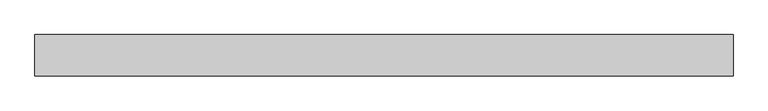
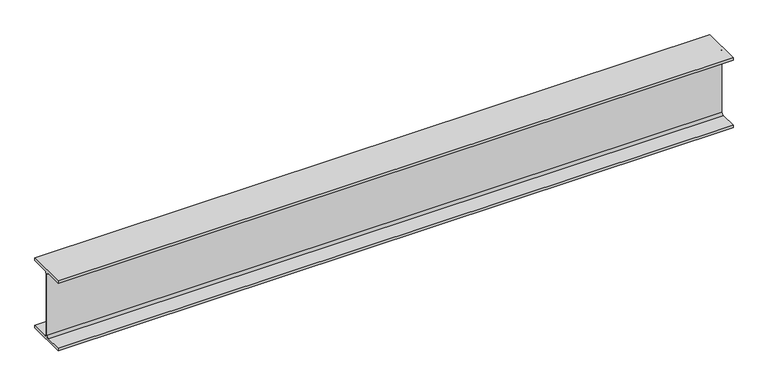
"""IFC4 building model written with IfcOpenShell, lengths in millimetres: beam geometry, Old_Steel Beam_H-KSD3502 : H_SB_ASB_H-250×125x6x9."""

from ifc_helpers import new_model, si_unit, point, frame, frame_2d, origin, place, context, project, spatial, polyline, circle_curve, trimmed, segment, composite_curve, outline, extrude, source, transform, mapped, element, save


def beam_a866aaba(model_context):
    return source(origin(), model_context, "Body", "SweptSolid", [
        extrude(outline(composite_curve([segment(polyline([(82.5, -141.5), (82.5, -151.7), (-82.5, -151.7), (-82.5, -141.5), (-11.9, -141.5)]), True, "CONTINUOUS"), segment(trimmed(circle_curve(frame_2d((-11.9, -132.6)), 8.9), [point((-11.9, -141.5))], [point((-3.0, -132.6))], True, "CARTESIAN"), True, "CONTINUOUS"), segment(polyline([(-3.0, -132.6), (-3.0, 132.6)]), True, "CONTINUOUS"), segment(trimmed(circle_curve(frame_2d((-11.9, 132.6)), 8.9), [point((-3.0, 132.6))], [point((-11.9, 141.5))], True, "CARTESIAN"), True, "CONTINUOUS"), segment(polyline([(-11.9, 141.5), (-82.5, 141.5), (-82.5, 151.7), (82.5, 151.7), (82.5, 141.5), (11.9, 141.5)]), True, "CONTINUOUS"), segment(trimmed(circle_curve(frame_2d((11.9, 132.6)), 8.9), [point((11.9, 141.5))], [point((3.0, 132.6))], True, "CARTESIAN"), True, "CONTINUOUS"), segment(polyline([(3.0, 132.6), (3.0, -132.6)]), True, "CONTINUOUS"), segment(trimmed(circle_curve(frame_2d((11.9, -132.6)), 8.9), [point((3.0, -132.6))], [point((11.9, -141.5))], True, "CARTESIAN"), True, "CONTINUOUS"), segment(polyline([(11.9, -141.5), (82.5, -141.5)]), True, "CONTINUOUS")], self_intersect=False)), frame((-1387.3, 0.0, 0.0), z_axis=(1.0, 0.0, 0.0), x_axis=(0.0, 1.0, 0.0)), (0.0, 0.0, 1.0), 2774.6),
    ])


if __name__ == "__main__":
    model = new_model("IFC4")
    model_context = context("Model", 3, world=origin())
    ifc_project = project(units=[si_unit("LENGTHUNIT", "METRE", prefix="MILLI")], contexts=[model_context])
    site = spatial("IfcSite", under=ifc_project)
    building = spatial("IfcBuilding", under=site)
    placement = place(None, origin())
    beam_shape = beam_a866aaba(model_context)
    element("IfcBeam", 1, ObjectType="Old_Steel Beam_H-KSD3502 : H_SB_ASB_H-250×125x6x9", at=placement, inside=building, context=model_context, shape_type="MappedRepresentation", body=[
        mapped(beam_shape, transform((0.0, 0.0, 0.0), x_axis=(1.0, 0.0, 0.0), y_axis=(0.0, 1.0, 0.0), z_axis=(0.0, 0.0, 1.0))),
    ])
    save(model, "model.ifc")

# Revit data of these elements
# Type "Old_Steel Beam_H-KSD3502 : H_SB_ASB_H-250×125x6x9"
#   Width = 12.5 cm
#   Web Thickness = 0.6 cm
#   Web Fillet = 1.2 cm
#   Warping Constant = 42539.8 cm⁶
#   Torsional Moment of Inertia = 7.8102 cm⁴
#   Torsional Modulus = 1.0 cm³
#   Section Area = 37.66 cm²
#   Plastic Modulus weak axis = 73.1 cm³
#   Plastic Modulus strong axis = 366.0 cm³
#   Perimeter = 0.97 m²/m
#   Nominal Weight = 29.60 kgf/m
#   Moment of Inertia weak axis = 294.00 cm⁴
#   Moment of Inertia strong axis = 4050.00 cm⁴
#   Height = 25.0 cm
#   Flange Thickness = 0.9 cm
#   Elastic Modulus weak axis = 47.0 cm³
#   Elastic Modulus strong axis = 324.0 cm³
#   Centroid Vertical = 12.5 cm
#   Centroid Horizontal = 6.25 cm
#   Length [instance default] = 1.5240 m
#   Structural Material [instance default] = Steel, 45-345
#   Assembly Code = ""
# Element 1 (IfcBeam, "Old_Steel Beam_H-KSD3502 : H_SB_ASB_H-250×125x6x9")
#   Structural Material = none
# Materials
#   "Steel, 45-345": class "Metal", colour RGB 189 187 185, transparency 0, Description = "Steel 345 MPa", Cost = 0
